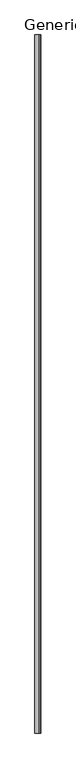
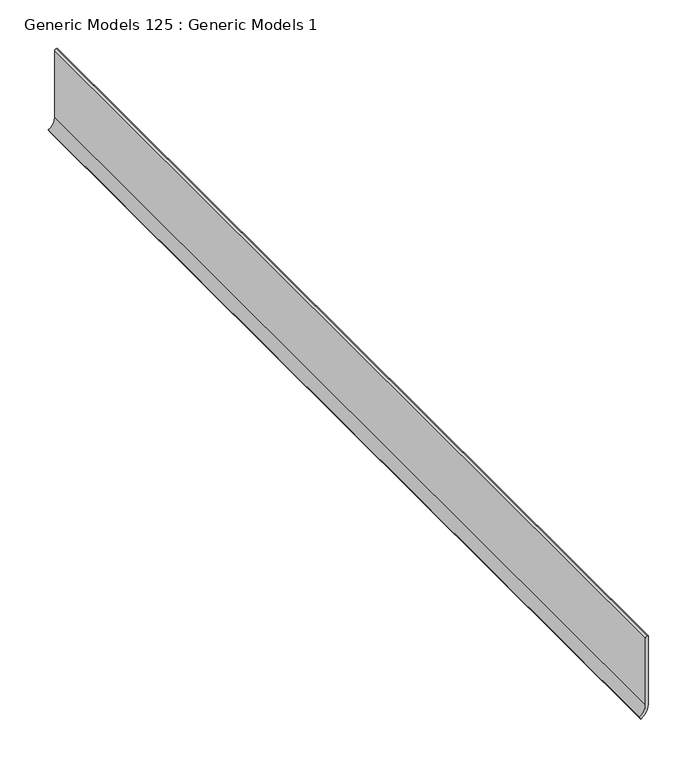
"""IFC4 building model written with IfcOpenShell, lengths in millimetres: proxy geometry, Generic Models 125 : Generic Models 1."""

from ifc_helpers import new_model, si_unit, point, frame, frame_2d, origin, place, context, project, spatial, polyline, circle_curve, trimmed, segment, composite_curve, outline, extrude, source, transform, mapped, element, save


def generic_models_125_generic_models_1_7d855ab6(model_context):
    return source(origin(), model_context, "Body", "SweptSolid", [
        extrude(outline(composite_curve([segment(polyline([(-2048.8233876, 49694.3681639), (-2048.8233876, 49693.2799657)]), True, "CONTINUOUS"), segment(trimmed(circle_curve(frame_2d((-2050.9101894, 49693.2799657)), 2.0868018), [point((-2048.8233876, 49693.2799657))], [point((-2050.9101894, 49691.1931639))], False, "CARTESIAN"), True, "CONTINUOUS"), segment(polyline([(-2050.9101894, 49691.1931639), (-2134.9737569, 49691.1931639)]), True, "CONTINUOUS"), segment(trimmed(circle_curve(frame_2d((-2134.9737569, 49676.528467)), 14.6646968), [point((-2134.9737569, 49691.1931639))], [point((-2147.6737569, 49683.8608155))], True, "CARTESIAN"), True, "CONTINUOUS"), segment(polyline([(-2147.6737569, 49683.8608155), (-2150.4233876, 49685.4483155)]), True, "CONTINUOUS"), segment(trimmed(circle_curve(frame_2d((-2134.9737569, 49676.528467)), 17.8396968), [point((-2150.4233876, 49685.4483155))], [point((-2134.9737569, 49694.3681639))], False, "CARTESIAN"), True, "CONTINUOUS"), segment(polyline([(-2134.9737569, 49694.3681639), (-2048.8233876, 49694.3681639)]), True, "CONTINUOUS")], self_intersect=False)), frame((0.0, 0.0, 0.0), z_axis=(0.0, 1.0, 0.0), x_axis=(0.0, 0.0, 1.0)), (0.0, 0.0, 1.0), 1219.2),
    ])


if __name__ == "__main__":
    model = new_model("IFC4")
    model_context = context("Model", 3, world=origin())
    ifc_project = project(units=[si_unit("LENGTHUNIT", "METRE", prefix="MILLI")], contexts=[model_context])
    site = spatial("IfcSite", under=ifc_project)
    building = spatial("IfcBuilding", under=site)
    placement = place(None, origin())
    generic_models_125_generic_models_1_shape = generic_models_125_generic_models_1_7d855ab6(model_context)
    element("IfcBuildingElementProxy", 1, Name="Generic Models 125 : Generic Models 1", ObjectType="Generic Models 125 : Generic Models 1", at=placement, inside=building, context=model_context, shape_type="MappedRepresentation", body=[
        mapped(generic_models_125_generic_models_1_shape, transform((0.0, 0.0, 0.0), x_axis=(1.0, 0.0, 0.0), y_axis=(0.0, 1.0, 0.0), z_axis=(0.0, 0.0, 1.0))),
    ])
    save(model, "model.ifc")

# Revit data of these elements
# Element 1 (IfcBuildingElementProxy, "Generic Models 125 : Generic Models 1")
#   Materials on its faces: "BASE T.B.D."
# Materials
#   "BASE T.B.D.": class "Generic", colour RGB 120 120 120, transparency 0, Cost = 0
